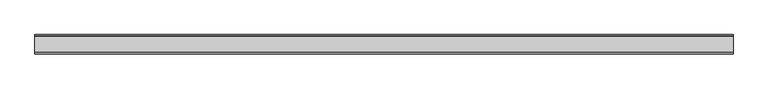
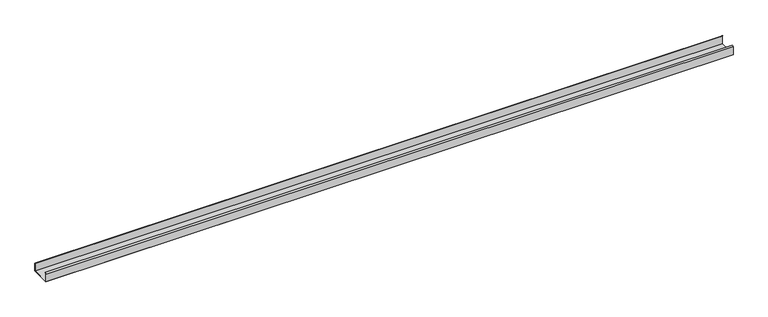
"""IFC4 building model written with IfcOpenShell, lengths in millimetres: proxy geometry, Generic Models 7:Generic Models 1:1:Generic Models 1:1 : Generic Models 7:Generic Models 1:337419:4 : Generic Models 7:Generic Models 1:1:Generic Models 1:1 : Generic Models 7:Generic Models 1:337419:306201."""

from ifc_helpers import new_model, si_unit, frame, origin, place, context, project, spatial, polyline, outline, extrude, source, transform, mapped, element, save


def generic_models_61b8e13d(model_context):
    return source(origin(), model_context, "Body", "SweptSolid", [
        extrude(outline(polyline([(-578797.4913841, 2446.5359375), (-579000.6913841, 2446.5359375), (-579000.6913841, 2535.4359375), (-578986.0982375, 2547.6810414), (-578984.3124931, 2545.5528742), (-578997.9132591, 2534.1404765), (-578997.9132591, 2449.3140625), (-578800.2695091, 2449.3140625), (-578800.2695091, 2534.1404765), (-578813.8702751, 2545.5528742), (-578812.0845307, 2547.6810414), (-578797.4913841, 2535.4359375), (-578797.4913841, 2446.5359375)])), frame((588867.6367239, 0.0, 0.0), z_axis=(1.0, 0.0, 0.0), x_axis=(0.0, 1.0, 0.0)), (0.0, 0.0, 1.0), 7315.2),
    ])


if __name__ == "__main__":
    model = new_model("IFC4")
    model_context = context("Model", 3, world=origin())
    ifc_project = project(units=[si_unit("LENGTHUNIT", "METRE", prefix="MILLI")], contexts=[model_context])
    site = spatial("IfcSite", under=ifc_project)
    building = spatial("IfcBuilding", under=site)
    placement = place(None, origin())
    generic_models_shape = generic_models_61b8e13d(model_context)
    element("IfcBuildingElementProxy", 1, Name="Generic Models 7:Generic Models 1:1:Generic Models 1:1 : Generic Models 7:Generic Models 1:337419:4 : Generic Models 7:Generic Models 1:1:Generic Models 1:1 : Generic Models 7:Generic Models 1:337419:306201", ObjectType="Generic Models 7:Generic Models 1:1:Generic Models 1:1 : Generic Models 7:Generic Models 1:337419:4 : Generic Models 7:Generic Models 1:1:Generic Models 1:1 : Generic Models 7:Generic Models 1:337419:306201", at=placement, inside=building, context=model_context, shape_type="MappedRepresentation", body=[
        mapped(generic_models_shape, transform((0.0, 0.0, 0.0), x_axis=(1.0, 0.0, 0.0), y_axis=(0.0, 1.0, 0.0), z_axis=(0.0, 0.0, 1.0))),
    ])
    save(model, "model.ifc")

# Revit data of these elements
# Type "Generic Models 7:Generic Models 1:1:Generic Models 1:1 : Generic Models 7:Generic Models 1:337419:4 : Generic Models 7:Generic Models 1:1:Generic Models 1:1 : Generic Models 7:Generic Models 1:337419:306201"
#   NameOverride = "Generic Models 7:Generic Models 1:1:Generic Models 1:1 : Generic Models 7:Generic Models 1:337419:306201"
#   ObjectTypeOverride = "Generic Models 1:1 : Generic Models 7:Generic Models 1:337419"
#   Reference = "Generic Models 1"
#   Tag = "306201"
# Element 1 (IfcBuildingElementProxy, "Generic Models 7:Generic Models 1:1:Generic Models 1:1 : Generic Models 7:Generic Models 1:337419:4 : Generic Models 7:Generic Models 1:1:Generic Models 1:1 : Generic Models 7:Generic Models 1:337419:306201")
#   Materials on its faces: "CEE' SECTION (8.0x3.5C - SEE STRUCT. DWGS)"
# Materials
#   "CEE' SECTION (8.0x3.5C - SEE STRUCT. DWGS)": class "Unassigned", colour RGB 210 209 208, transparency 0, Keynote = "M05121300.02", Cost = 0
